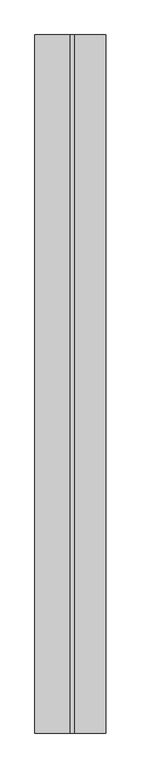
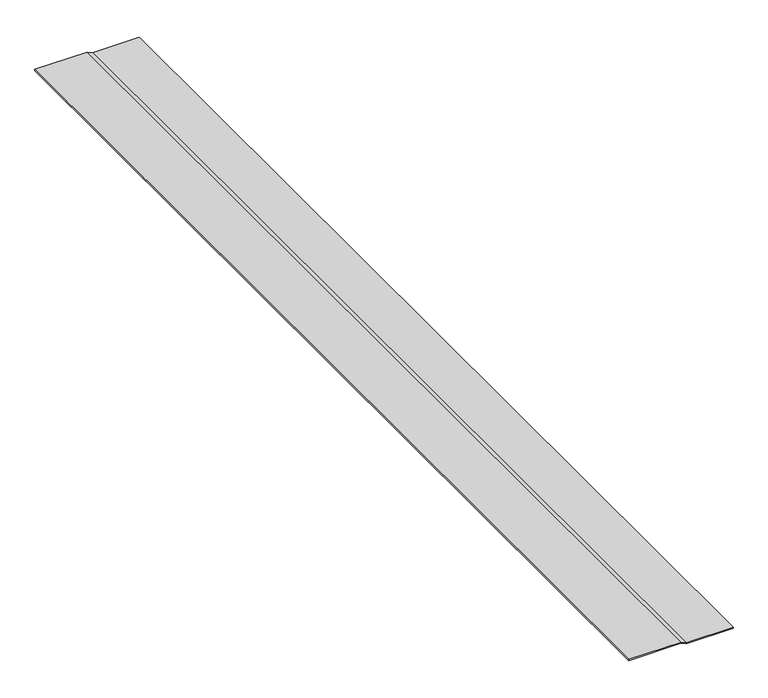
"""IFC4 building model written with IfcOpenShell, lengths in millimetres: proxy geometry, INTERPLY001 : INTERPLY001."""

from ifc_helpers import new_model, si_unit, frame, origin, place, context, project, spatial, polyline, outline, extrude, source, transform, mapped, element, save


def generic_models_0b97792e(model_context):
    return source(origin(), model_context, "Body", "SweptSolid", [
        extrude(outline(polyline([(40265.8733085, -4907.7318464), (40265.8733085, -5009.4682358), (40263.5642176, -5009.4682358), (40263.5642176, -4908.2233377), (40258.8529944, -4897.657757), (40258.8529944, -4806.4281968), (40261.1620854, -4806.4281968), (40261.1620854, -4897.1662657), (40265.8733085, -4907.7318464)])), frame((0.0, -1052.8906574, 0.0), z_axis=(0.0, 1.0, 0.0), x_axis=(0.0, 0.0, 1.0)), (0.0, 0.0, 1.0), 2000.25),
    ])


if __name__ == "__main__":
    model = new_model("IFC4")
    model_context = context("Model", 3, world=origin())
    ifc_project = project(units=[si_unit("LENGTHUNIT", "METRE", prefix="MILLI")], contexts=[model_context])
    site = spatial("IfcSite", under=ifc_project)
    building = spatial("IfcBuilding", under=site)
    placement = place(None, origin())
    generic_models_shape = generic_models_0b97792e(model_context)
    element("IfcBuildingElementProxy", 1, Name="INTERPLY001 : INTERPLY001", ObjectType="INTERPLY001 : INTERPLY001", at=placement, inside=building, context=model_context, shape_type="MappedRepresentation", body=[
        mapped(generic_models_shape, transform((0.0, 0.0, 0.0), x_axis=(1.0, 0.0, 0.0), y_axis=(0.0, 1.0, 0.0), z_axis=(0.0, 0.0, 1.0))),
    ])
    save(model, "model.ifc")

# Revit data of these elements
# Type "INTERPLY001 : INTERPLY001"
#   NameOverride = "INTERPLY001"
# Element 1 (IfcBuildingElementProxy, "INTERPLY001 : INTERPLY001")
#   Materials on its faces: "INTERPLY REQUIRED FOR 15 & 20 YEARS SYSTEMS"
# Materials
#   "INTERPLY REQUIRED FOR 15 & 20 YEARS SYSTEMS": class "Unassigned", colour RGB 115 115 172, transparency 0
